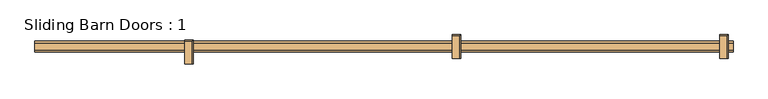
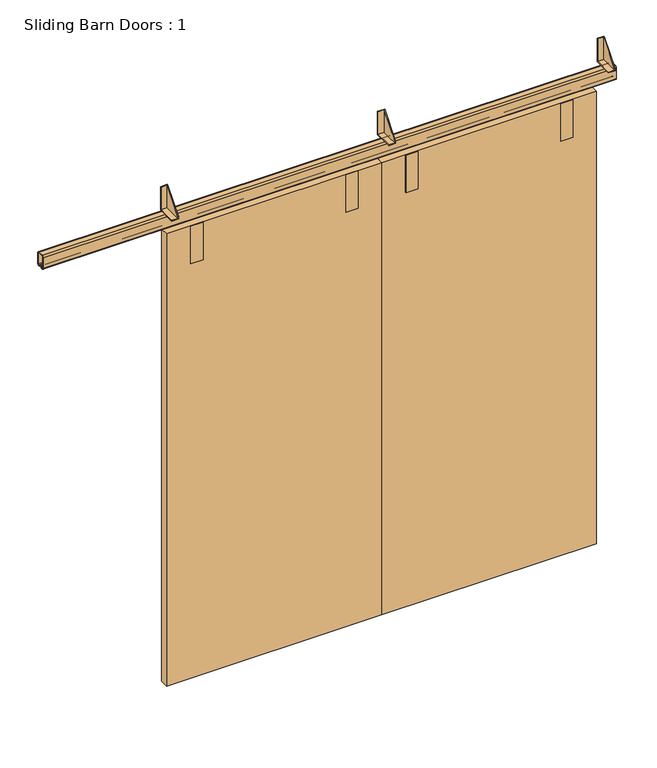
"""IFC4 building model written with IfcOpenShell, lengths in millimetres: door geometry, Sliding Barn Doors : 1."""

from ifc_helpers import new_model, si_unit, point, frame, frame_2d, origin, place, context, project, spatial, polyline, circle_curve, trimmed, segment, composite_curve, outline, extrude, source, transform, mapped, element, save


def sliding_barn_doors_1_1aa09791(model_context):
    return source(origin(), model_context, "Body", "SweptSolid", [
        extrude(outline(polyline([(-158.75, 2152.65), (-79.375, 2247.773), (-79.375, 2146.3), (-158.75, 2146.3), (-158.75, 2152.65)])), frame((-1418.4808594, 0.0, 0.0), z_axis=(1.0, 0.0, 0.0), x_axis=(0.0, 1.0, 0.0)), (0.0, 0.0, 1.0), 3.175),
        extrude(outline(polyline([(-76.2, 2143.125), (-158.75, 2143.125), (-158.75, 2146.3), (-79.375, 2146.3), (-79.375, 2247.773), (-76.2, 2247.773), (-76.2, 2143.125)])), frame((-1443.7816406, 0.0, 0.0), z_axis=(1.0, 0.0, 0.0), x_axis=(0.0, 1.0, 0.0)), (0.0, 0.0, 1.0), 28.4757812),
        extrude(outline(polyline([(-139.7, 2152.65), (-60.325, 2247.773), (-60.325, 2146.3), (-139.7, 2146.3), (-139.7, 2152.65)])), frame((-484.2371094, 0.0, 0.0), z_axis=(1.0, 0.0, 0.0), x_axis=(0.0, 1.0, 0.0)), (0.0, 0.0, 1.0), 3.175),
        extrude(outline(polyline([(-57.15, 2143.125), (-139.7, 2143.125), (-139.7, 2146.3), (-60.325, 2146.3), (-60.325, 2247.773), (-57.15, 2247.773), (-57.15, 2143.125)])), frame((-509.5378906, 0.0, 0.0), z_axis=(1.0, 0.0, 0.0), x_axis=(0.0, 1.0, 0.0)), (0.0, 0.0, 1.0), 28.4757813),
        extrude(outline(polyline([(-139.7, 2152.65), (-60.325, 2247.773), (-60.325, 2146.3), (-139.7, 2146.3), (-139.7, 2152.65)])), frame((450.0066406, 0.0, 0.0), z_axis=(1.0, 0.0, 0.0), x_axis=(0.0, 1.0, 0.0)), (0.0, 0.0, 1.0), 3.175),
        extrude(outline(polyline([(-57.15, 2143.125), (-139.7, 2143.125), (-139.7, 2146.3), (-60.325, 2146.3), (-60.325, 2247.773), (-57.15, 2247.773), (-57.15, 2143.125)])), frame((424.7058594, 0.0, 0.0), z_axis=(1.0, 0.0, 0.0), x_axis=(0.0, 1.0, 0.0)), (0.0, 0.0, 1.0), 28.4757813),
        extrude(outline(polyline([(-1339.31025, -117.475), (-1339.31025, -114.3), (-1288.00225, -114.3), (-1288.00225, -117.475), (-1339.31025, -117.475)])), frame((0.0, 0.0, 1889.252), z_axis=(0.0, 0.0, 1.0), x_axis=(1.0, 0.0, 0.0)), (0.0, 0.0, 1.0), 168.148),
        extrude(outline(polyline([(-678.91025, -117.475), (-678.91025, -114.3), (-627.60225, -114.3), (-627.60225, -117.475), (-678.91025, -117.475)])), frame((0.0, 0.0, 1889.252), z_axis=(0.0, 0.0, 1.0), x_axis=(1.0, 0.0, 0.0)), (0.0, 0.0, 1.0), 168.148),
        extrude(outline(polyline([(-424.91025, -117.475), (-424.91025, -114.3), (-373.60225, -114.3), (-373.60225, -117.475), (-424.91025, -117.475)])), frame((0.0, 0.0, 1889.252), z_axis=(0.0, 0.0, 1.0), x_axis=(1.0, 0.0, 0.0)), (0.0, 0.0, 1.0), 168.148),
        extrude(outline(polyline([(235.48975, -117.475), (235.48975, -114.3), (286.79775, -114.3), (286.79775, -117.475), (235.48975, -117.475)])), frame((0.0, 0.0, 1889.252), z_axis=(0.0, 0.0, 1.0), x_axis=(1.0, 0.0, 0.0)), (0.0, 0.0, 1.0), 168.148),
        extrude(outline(polyline([(-1440.65625, -114.3), (-1440.65625, -79.375), (-526.25625, -79.375), (-526.25625, -114.3), (-1440.65625, -114.3)])), frame((0.0, 0.0, 25.4), z_axis=(0.0, 0.0, 1.0), x_axis=(1.0, 0.0, 0.0)), (0.0, 0.0, 1.0), 2032.0),
        extrude(outline(polyline([(-526.25625, -114.3), (-526.25625, -79.375), (388.14375, -79.375), (388.14375, -114.3), (-526.25625, -114.3)])), frame((0.0, 0.0, 25.4), z_axis=(0.0, 0.0, 1.0), x_axis=(1.0, 0.0, 0.0)), (0.0, 0.0, 1.0), 2032.0),
        extrude(outline(composite_curve([segment(trimmed(circle_curve(frame_2d((-85.725, 2136.775)), 6.35), [point((-85.725, 2143.125))], [point((-79.375, 2136.775))], False, "CARTESIAN"), True, "CONTINUOUS"), segment(polyline([(-79.375, 2136.775), (-79.375, 2088.515)]), True, "CONTINUOUS"), segment(trimmed(circle_curve(frame_2d((-85.725, 2088.515)), 6.35), [point((-79.375, 2088.515))], [point((-85.725, 2082.165))], False, "CARTESIAN"), True, "CONTINUOUS"), segment(polyline([(-85.725, 2082.165), (-91.1336853, 2082.165)]), True, "CONTINUOUS"), segment(trimmed(circle_curve(frame_2d((-91.1336853, 2083.7525)), 1.5875), [point((-91.1336853, 2082.165))], [point((-92.6920184, 2083.4495907))], False, "CARTESIAN"), True, "CONTINUOUS"), segment(polyline([(-92.6920184, 2083.4495907), (-94.1175341, 2090.7832331), (-92.6013971, 2090.7832331), (-91.2154749, 2083.6532812), (-85.725, 2083.6532812)]), True, "CONTINUOUS"), segment(trimmed(circle_curve(frame_2d((-85.725, 2088.515)), 4.8617187), [point((-85.725, 2083.6532812))], [point((-80.8632813, 2088.515))], True, "CARTESIAN"), True, "CONTINUOUS"), segment(polyline([(-80.8632813, 2088.515), (-80.8632813, 2136.775)]), True, "CONTINUOUS"), segment(trimmed(circle_curve(frame_2d((-85.725, 2136.775)), 4.8617187), [point((-80.8632813, 2136.775))], [point((-85.725, 2141.6367187))], True, "CARTESIAN"), True, "CONTINUOUS"), segment(polyline([(-85.725, 2141.6367187), (-111.252, 2141.6367187)]), True, "CONTINUOUS"), segment(trimmed(circle_curve(frame_2d((-111.252, 2136.775)), 4.8617187), [point((-111.252, 2141.6367187))], [point((-116.1137188, 2136.775))], True, "CARTESIAN"), True, "CONTINUOUS"), segment(polyline([(-116.1137188, 2136.775), (-116.1137188, 2088.515)]), True, "CONTINUOUS"), segment(trimmed(circle_curve(frame_2d((-111.252, 2088.515)), 4.8617187), [point((-116.1137188, 2088.515))], [point((-111.252, 2083.6532812))], True, "CARTESIAN"), True, "CONTINUOUS"), segment(polyline([(-111.252, 2083.6532812), (-105.7615251, 2083.6532812), (-104.3756029, 2090.7832331), (-102.8594659, 2090.7832331), (-104.2849816, 2083.4495907)]), True, "CONTINUOUS"), segment(trimmed(circle_curve(frame_2d((-105.8433147, 2083.7525)), 1.5875), [point((-104.2849816, 2083.4495907))], [point((-105.8433147, 2082.165))], False, "CARTESIAN"), True, "CONTINUOUS"), segment(polyline([(-105.8433147, 2082.165), (-111.252, 2082.165)]), True, "CONTINUOUS"), segment(trimmed(circle_curve(frame_2d((-111.252, 2088.515)), 6.35), [point((-111.252, 2082.165))], [point((-117.602, 2088.515))], False, "CARTESIAN"), True, "CONTINUOUS"), segment(polyline([(-117.602, 2088.515), (-117.602, 2136.775)]), True, "CONTINUOUS"), segment(trimmed(circle_curve(frame_2d((-111.252, 2136.775)), 6.35), [point((-117.602, 2136.775))], [point((-111.252, 2143.125))], False, "CARTESIAN"), True, "CONTINUOUS"), segment(polyline([(-111.252, 2143.125), (-85.725, 2143.125)]), True, "CONTINUOUS")], self_intersect=False)), frame((-1967.70625, 0.0, 0.0), z_axis=(1.0, 0.0, 0.0), x_axis=(0.0, 1.0, 0.0)), (0.0, 0.0, 1.0), 2438.4),
    ])


if __name__ == "__main__":
    model = new_model("IFC4")
    model_context = context("Model", 3, world=origin())
    ifc_project = project(units=[si_unit("LENGTHUNIT", "METRE", prefix="MILLI")], contexts=[model_context])
    site = spatial("IfcSite", under=ifc_project)
    building = spatial("IfcBuilding", under=site)
    placement = place(None, origin())
    sliding_barn_doors_1_shape = sliding_barn_doors_1_1aa09791(model_context)
    element("IfcDoor", 1, ObjectType="Sliding Barn Doors : 1", at=placement, inside=building, context=model_context, shape_type="MappedRepresentation", body=[
        mapped(sliding_barn_doors_1_shape, transform((0.0, 0.0, 0.0), x_axis=(1.0, 0.0, 0.0), y_axis=(0.0, 1.0, 0.0), z_axis=(0.0, 0.0, 1.0))),
    ])
    save(model, "model.ifc")

# Revit data of these elements
# Type "Sliding Barn Doors : 1"
#   Type Mark = "26"
#   Analytic Construction = "<None>"
#   rail_overlap_left = 0' - 5 1/4"
#   rail_length = 8' - 0"
#   overlap_left = 0' - 2"
#   overlap = 0' - 0"
#   bracket_right = 3' - 7"
#   bracket_left = 0' - 4"
#   Thickness = 0' - 1 3/8"
#   Panel Width = 3' - 0"
#   Panel Height = 6' - 8"
#   Gap 2 = 0' - 0 1/2"
#   Gap 1 = 0' - 0 7/8"
#   Frame Projection Ext. = 0' - 1"
#   Frame Projection Int. = 0' - 1"
#   Frame Width = 0' - 3"
#   Height = 6' - 4"
#   Width = 2' - 2 9/16"
#   Bracket_offset = 0' - 5"
#   Door_4 = no
#   Door_3 = no
#   Hardware Material = Metal - Aluminum
#   Door Material = Closet_1
#   Function = (empty or 0)
#   Wall Closure = (empty or 0)
# Element 1 (IfcDoor, "Sliding Barn Doors : 1")
#   Materials on its faces: "Metal - Aluminum", "Closet_1"
# Materials
#   "Metal - Aluminum": class "Metal", colour RGB 247 247 247, transparency 0
#   "Closet_1": class "Paint", colour RGB 58 62 47, transparency 0, Cost = 0
